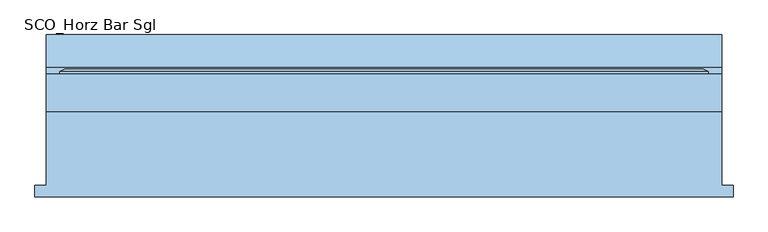
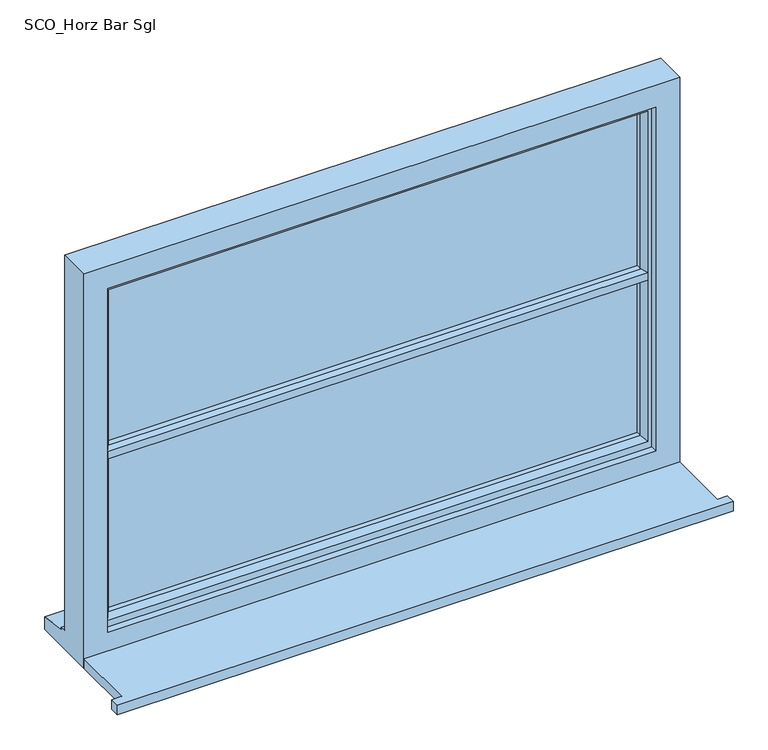
"""IFC4 building model written with IfcOpenShell, lengths in millimetres: window geometry, SCO_Horz Bar Sgl : SCO_Horz Bar Sgl G.F."""

from ifc_helpers import new_model, si_unit, frame, origin, place, context, project, spatial, polyline, outline, extrude, faceted_brep, source, transform, mapped, element, save


def sco_horz_bar_sgl_0312c325(model_context):
    return source(origin(), model_context, "Body", "SolidModel", [
        extrude(outline(polyline([(-775.0, -191.5434322), (-775.0, -166.5434322), (-750.0, -166.5434322), (-750.0, -2.0434322), (750.0, -2.0434322), (750.0, -166.5434322), (775.0, -166.5434322), (775.0, -191.5434322), (-775.0, -191.5434322)])), frame((0.0, 0.0, 1060.0), z_axis=(0.0, 0.0, 1.0), x_axis=(1.0, 0.0, 0.0)), (0.0, 0.0, 1.0), 25.0),
        faceted_brep([(-750.0, -2.0434322, 1060.0), (750.0, -2.0434322, 1060.0), (750.0, -2.0434322, 2110.0), (-750.0, -2.0434322, 2110.0), (-690.0, -2.0434322, 2050.0), (690.0, -2.0434322, 2050.0), (690.0, -2.0434322, 1135.0), (-690.0, -2.0434322, 1135.0), (-750.0, 80.9565678, 2110.0), (-750.0, 80.9565678, 1111.0), (-750.0, 95.9565678, 1109.68767), (-750.0, 95.9565678, 1104.7449676), (-750.0, 168.4565678, 1093.8088847), (-750.0, 168.4565678, 1060.0), (750.0, 80.9565678, 2110.0), (750.0, 80.9565678, 1111.0), (-710.0, 80.9565678, 2070.0), (-710.0, 80.9565678, 1123.0), (710.0, 80.9565678, 1123.0), (710.0, 80.9565678, 2070.0), (-710.0, 15.9565678, 2070.0), (-710.0, 15.9565678, 1123.0), (710.0, 15.9565678, 2070.0), (710.0, 15.9565678, 1123.0), (-690.0, 15.9565678, 2050.0), (-690.0, 15.9565678, 1135.0), (690.0, 15.9565678, 1135.0), (690.0, 15.9565678, 2050.0), (750.0, 168.4565678, 1060.0), (750.0, 168.4565678, 1093.8088847), (750.0, 95.9565678, 1104.7449676), (750.0, 95.9565678, 1109.68767)], [[[0, 1, 2, 3], [4, 5, 6, 7]], [[0, 3, 8, 9, 10, 11, 12, 13]], [[9, 8, 14, 15], [16, 17, 18, 19]], [[17, 16, 20, 21]], [[20, 22, 23, 21], [24, 25, 26, 27]], [[24, 4, 7, 25]], [[3, 2, 14, 8]], [[16, 19, 22, 20]], [[5, 4, 24, 27]], [[15, 14, 2, 1, 28, 29, 30, 31]], [[19, 18, 23, 22]], [[5, 27, 26, 6]], [[28, 1, 0, 13]], [[29, 28, 13, 12]], [[30, 29, 12, 11]], [[31, 30, 11, 10]], [[15, 31, 10, 9]], [[21, 23, 18, 17]], [[7, 6, 26, 25]]]),
        extrude(outline(polyline([(680.1480377, 44.9565678), (-680.0, 44.9565678), (-680.0, 68.9565678), (680.1480377, 68.9565678), (680.1480377, 44.9565678)])), frame((0.0, 0.0, 1153.0), z_axis=(0.0, 0.0, 1.0), x_axis=(1.0, 0.0, 0.0)), (0.0, 0.0, 1.0), 434.3307627),
        extrude(outline(polyline([(680.1480377, 44.9565678), (-680.0, 44.9565678), (-680.0, 68.9565678), (680.1480377, 68.9565678), (680.1480377, 44.9565678)])), frame((0.0, 0.0, 1597.6692373), z_axis=(0.0, 0.0, 1.0), x_axis=(1.0, 0.0, 0.0)), (0.0, 0.0, 1.0), 442.3307627),
        extrude(outline(polyline([(92.5035732, 1597.6692373), (92.5035732, 1587.3307627), (86.8277797, 1577.5), (68.9565678, 1577.5), (68.9565678, 1584.5), (44.9565678, 1584.5), (44.9565678, 1577.5), (30.4494677, 1577.5), (15.9565678, 1582.6480377), (15.9565678, 1602.3519623), (30.4494677, 1607.5), (44.9565678, 1607.5), (44.9565678, 1600.5), (68.9565678, 1600.5), (68.9565678, 1607.5), (86.8277797, 1607.5), (92.5035732, 1597.6692373)])), frame((-680.1480377, 0.0, 0.0), z_axis=(1.0, 0.0, 0.0), x_axis=(0.0, 1.0, 0.0)), (0.0, 0.0, 1.0), 1360.2960754),
        faceted_brep([(-720.0, 80.9565678, 2072.0), (-720.0, 86.7300705, 2072.0), (-720.0, 86.7300705, 1113.0), (-720.0, 80.9565678, 1113.0), (-710.0, 15.9565678, 2062.0), (-710.0, 80.9565678, 2062.0), (-710.0, 80.9565678, 1123.0), (-710.0, 15.9565678, 1123.0), (-670.0, 30.4494677, 2022.0), (-680.1480377, 15.9565678, 2032.1480377), (-680.1480377, 15.9565678, 1152.8519623), (-670.0, 30.4494677, 1163.0), (-670.0, 44.9565678, 2022.0), (-670.0, 44.9565678, 1163.0), (-680.0, 68.9565678, 2032.0), (-680.0, 44.9565678, 2032.0), (-680.0, 44.9565678, 1153.0), (-680.0, 68.9565678, 1153.0), (-670.0, 86.7300705, 2022.0), (-670.0, 68.9565678, 2022.0), (-670.0, 68.9565678, 1163.0), (-670.0, 86.7300705, 1163.0), (-680.0, 92.5035732, 2032.0), (-680.0, 92.5035732, 1153.0), (-709.2153903, 92.5035732, 2061.2153903), (-709.2153903, 92.5035732, 1123.7846097), (720.0, 86.7300705, 1113.0), (720.0, 80.9565678, 1113.0), (710.0, 80.9565678, 1123.0), (710.0, 15.9565678, 1123.0), (680.1480377, 15.9565678, 1152.8519623), (670.0, 30.4494677, 1163.0), (670.0, 44.9565678, 1163.0), (680.0, 44.9565678, 1153.0), (680.0, 68.9565678, 1153.0), (670.0, 68.9565678, 1163.0), (670.0, 86.7300705, 1163.0), (680.0, 92.5035732, 1153.0), (709.2153903, 92.5035732, 1123.7846097), (720.0, 86.7300705, 2072.0), (720.0, 80.9565678, 2072.0), (710.0, 80.9565678, 2062.0), (710.0, 15.9565678, 2062.0), (680.1480377, 15.9565678, 2032.1480377), (670.0, 30.4494677, 2022.0), (670.0, 44.9565678, 2022.0), (680.0, 44.9565678, 2032.0), (680.0, 68.9565678, 2032.0), (670.0, 68.9565678, 2022.0), (670.0, 86.7300705, 2022.0), (680.0, 92.5035732, 2032.0), (709.2153903, 92.5035732, 2061.2153903)], [[[0, 1, 2, 3]], [[4, 5, 6, 7]], [[8, 9, 10, 11]], [[12, 8, 11, 13]], [[14, 15, 16, 17]], [[18, 19, 20, 21]], [[22, 18, 21, 23]], [[1, 24, 25, 2]], [[3, 2, 26, 27]], [[7, 6, 28, 29]], [[11, 10, 30, 31]], [[13, 11, 31, 32]], [[17, 16, 33, 34]], [[21, 20, 35, 36]], [[23, 21, 36, 37]], [[2, 25, 38, 26]], [[27, 26, 39, 40]], [[29, 28, 41, 42]], [[31, 30, 43, 44]], [[32, 31, 44, 45]], [[34, 33, 46, 47]], [[36, 35, 48, 49]], [[37, 36, 49, 50]], [[26, 38, 51, 39]], [[40, 39, 1, 0]], [[3, 27, 40, 0], [5, 41, 28, 6]], [[42, 41, 5, 4]], [[7, 29, 42, 4], [9, 43, 30, 10]], [[44, 43, 9, 8]], [[45, 44, 8, 12]], [[15, 46, 33, 16], [13, 32, 45, 12]], [[47, 46, 15, 14]], [[17, 34, 47, 14], [19, 48, 35, 20]], [[49, 48, 19, 18]], [[50, 49, 18, 22]], [[24, 51, 38, 25], [23, 37, 50, 22]], [[39, 51, 24, 1]]]),
    ])


if __name__ == "__main__":
    model = new_model("IFC4")
    model_context = context("Model", 3, world=origin())
    ifc_project = project(units=[si_unit("LENGTHUNIT", "METRE", prefix="MILLI")], contexts=[model_context])
    site = spatial("IfcSite", under=ifc_project)
    building = spatial("IfcBuilding", under=site)
    placement = place(None, origin())
    sco_horz_bar_sgl_shape = sco_horz_bar_sgl_0312c325(model_context)
    element("IfcWindow", 1, ObjectType="SCO_Horz Bar Sgl : SCO_Horz Bar Sgl G.F", at=placement, inside=building, context=model_context, shape_type="MappedRepresentation", body=[
        mapped(sco_horz_bar_sgl_shape, transform((0.0, 0.0, 0.0), x_axis=(1.0, 0.0, 0.0), y_axis=(0.0, 1.0, 0.0), z_axis=(0.0, 0.0, 1.0))),
    ])
    save(model, "model.ifc")

# Revit data of these elements
# Type "SCO_Horz Bar Sgl : SCO_Horz Bar Sgl G.F"
#   Type Mark = "W1"
#   Operation = "SinglePanel"
#   Manufacturer = "Revit"
#   Keynote = "L10"
#   Wrap Layers (Ext) from Ext = 102.5 mm
#   Wrap Layers (Int) from Ext = 177.5 mm
#   Window Board Projection = 25 mm
#   Window Board Extension = 25 mm
#   Rough Width = 1500 mm
#   Rough Height = 1050 mm
#   Height = 1050 mm
#   Width = 1500 mm
#   Glazing Thickness = 24 mm
#   FrameOffset - External = 102.5 mm
#   Frame Depth = 65 mm
#   Ext Leaf Thickness (Scot) = 102.5 mm
#   Ext Leaf Overlap (Scot) = 25 mm
#   Default Head Height = 2110 mm
#   Cill Depth = 87.5 mm
#   Cavity Closer Width = 50 mm
#   Cavity Closer Offset from Ext = 102.5 mm
#   Cavity Closer Depth = 85 mm
#   Vis - Cavity Closers = yes
#   Material Trim = Window Frame
#   Material Glass = Glass
#   Material Frame = Window Frame
#   Wall Closure = (empty or 0)
# Element 1 (IfcWindow, "SCO_Horz Bar Sgl : SCO_Horz Bar Sgl G.F")
#   Materials on its faces: "Window Frame", "Glass"
# Materials
#   "Window Frame": class "Miscellaneous", colour RGB 249 249 249, transparency 0
#   "Glass": class "Glass", colour RGB 0 128 192, transparency 0.75
